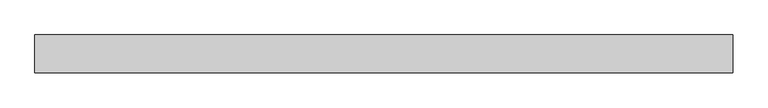
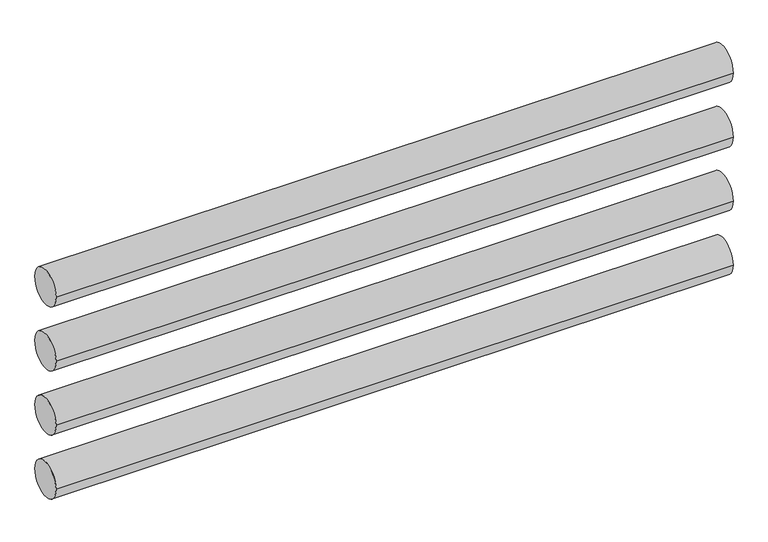
"""IFC4 building model written with IfcOpenShell, lengths in millimetres: proxy geometry, Газпремиум_Регистр : РГТ-1-108х3-2м-4."""

from ifc_helpers import new_model, si_unit, point, frame, frame_2d, origin, place, context, project, spatial, circle_curve, trimmed, segment, composite_curve, outline, extrude, source, transform, mapped, element, save


def mechanical_equipment_8a01154c(model_context):
    return source(origin(), model_context, "Body", "SweptSolid", [
        extrude(outline(composite_curve([segment(trimmed(circle_curve(frame_2d((0.0, 654.0)), 54.0), [point((-54.0, 654.0))], [point((54.0, 654.0))], False, "CARTESIAN"), True, "CONTINUOUS"), segment(trimmed(circle_curve(frame_2d((0.0, 654.0)), 54.0), [point((54.0, 654.0))], [point((-54.0, 654.0))], False, "CARTESIAN"), True, "CONTINUOUS")], self_intersect=False)), frame((-184.1719207, 0.0, 0.0), z_axis=(1.0, 0.0, 0.0), x_axis=(0.0, 1.0, 0.0)), (0.0, 0.0, 1.0), 2000.0),
        extrude(outline(composite_curve([segment(trimmed(circle_curve(frame_2d((0.0, 454.0)), 54.0), [point((-54.0, 454.0))], [point((54.0, 454.0))], False, "CARTESIAN"), True, "CONTINUOUS"), segment(trimmed(circle_curve(frame_2d((0.0, 454.0)), 54.0), [point((54.0, 454.0))], [point((-54.0, 454.0))], False, "CARTESIAN"), True, "CONTINUOUS")], self_intersect=False)), frame((-184.1719207, 0.0, 0.0), z_axis=(1.0, 0.0, 0.0), x_axis=(0.0, 1.0, 0.0)), (0.0, 0.0, 1.0), 2000.0),
        extrude(outline(composite_curve([segment(trimmed(circle_curve(frame_2d((0.0, 254.0)), 54.0), [point((-54.0, 254.0))], [point((54.0, 254.0))], False, "CARTESIAN"), True, "CONTINUOUS"), segment(trimmed(circle_curve(frame_2d((0.0, 254.0)), 54.0), [point((54.0, 254.0))], [point((-54.0, 254.0))], False, "CARTESIAN"), True, "CONTINUOUS")], self_intersect=False)), frame((-184.1719207, 0.0, 0.0), z_axis=(1.0, 0.0, 0.0), x_axis=(0.0, 1.0, 0.0)), (0.0, 0.0, 1.0), 2000.0),
        extrude(outline(composite_curve([segment(trimmed(circle_curve(frame_2d((0.0, 54.0)), 54.0), [point((-54.0, 54.0))], [point((54.0, 54.0))], False, "CARTESIAN"), True, "CONTINUOUS"), segment(trimmed(circle_curve(frame_2d((0.0, 54.0)), 54.0), [point((54.0, 54.0))], [point((-54.0, 54.0))], False, "CARTESIAN"), True, "CONTINUOUS")], self_intersect=False)), frame((-184.1719207, 0.0, 0.0), z_axis=(1.0, 0.0, 0.0), x_axis=(0.0, 1.0, 0.0)), (0.0, 0.0, 1.0), 2000.0),
    ])


if __name__ == "__main__":
    model = new_model("IFC4")
    model_context = context("Model", 3, world=origin())
    ifc_project = project(units=[si_unit("LENGTHUNIT", "METRE", prefix="MILLI")], contexts=[model_context])
    site = spatial("IfcSite", under=ifc_project)
    building = spatial("IfcBuilding", under=site)
    placement = place(None, origin())
    mechanical_equipment_shape = mechanical_equipment_8a01154c(model_context)
    element("IfcBuildingElementProxy", 1, Name="Газпремиум_Регистр : РГТ-1-108х3-2м-4", ObjectType="Газпремиум_Регистр : РГТ-1-108х3-2м-4", at=placement, inside=building, context=model_context, shape_type="MappedRepresentation", body=[
        mapped(mechanical_equipment_shape, transform((0.0, 0.0, 0.0), x_axis=(1.0, 0.0, 0.0), y_axis=(0.0, 1.0, 0.0), z_axis=(0.0, 0.0, 1.0))),
    ])
    save(model, "model.ifc")

# Revit data of these elements
# Type "Газпремиум_Регистр : РГТ-1-108х3-2м-4"
#   ADSK_Позиция = "387"
#   ADSK_Наименование = "Регистр однорядный из четырех гладких труб 108х3 длиной 2 м, в комплекте с опорами"
#   ADSK_Марка = "РГТ-1-108х3-2м-4-ОП-О ТУ 4936-001-69441315-11"
#   ADSK_Код изделия = "2050898"
#   ADSK_Завод-изготовитель = "ООО ПКП \"ГазПремиум\", Россия, г.Саратов, ИНН 6452951387, кпп 645201001, gaz-premium@mail.ru"
#   ADSK_Единица измерения = "шт."
#   Расстояние между рядами = 200 mm
#   Радиус.регистра = 54 mm
#   Отступ.труб.подкл.от.осевой = 32.719 mm
#   Длина регистра = 2000 mm
#   Диаметр.труб.подкл. = 32 mm
#   Диаметр регистра = 108 mm
#   Высота = 600 mm
#   ADSK_Масса = 79.31
#   ADSK_Количество = 1
#   Число рядов = 4
#   Соед.трубы = Грунтовка.красная
#   Регистр = Грунтовка.красная
#   Поддерж.арматура = Грунтовка.серая
#   Default Elevation = 0
# Element 1 (IfcBuildingElementProxy, "Газпремиум_Регистр : РГТ-1-108х3-2м-4")
#   Materials on its faces: "Грунтовка.красная"
# Materials
#   "Грунтовка.красная": class "Разное", colour RGB 255 0 0, transparency 0
#   "Грунтовка.серая": class "Разное", colour RGB 187 181 179, transparency 0
